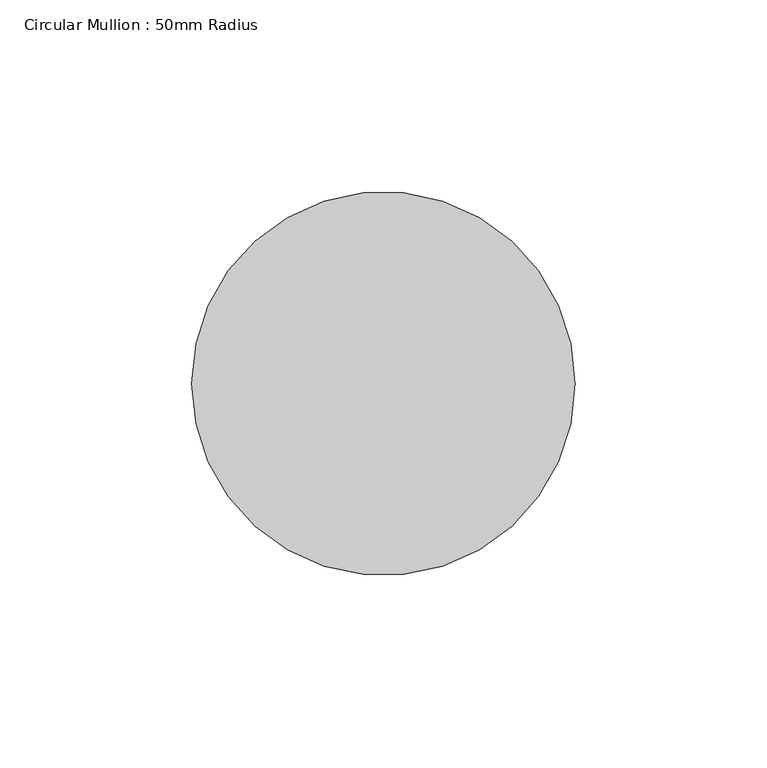
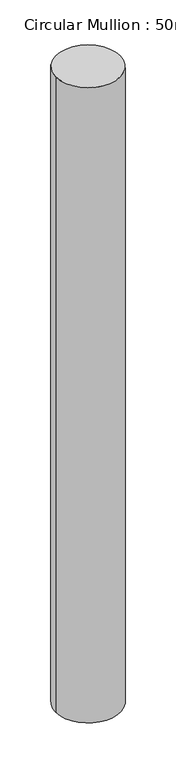
"""IFC4 building model written with IfcOpenShell, lengths in millimetres: member geometry, Circular Mullion : 50mm Radius."""

from ifc_helpers import new_model, si_unit, point, frame, origin, origin_2d, place, context, project, spatial, circle_curve, trimmed, segment, composite_curve, outline, extrude, source, transform, mapped, element, save


def circular_mullion_50mm_radius_1879a9a9(model_context):
    return source(origin(), model_context, "Body", "SweptSolid", [
        extrude(outline(composite_curve([segment(trimmed(circle_curve(origin_2d(), 50.0), [point((50.0, 0.0))], [point((-50.0, 0.0))], False, "CARTESIAN"), True, "CONTINUOUS"), segment(trimmed(circle_curve(origin_2d(), 50.0), [point((-50.0, 0.0))], [point((50.0, 0.0))], False, "CARTESIAN"), True, "CONTINUOUS")], self_intersect=False)), frame((0.0, 0.0, -1042.8045224), z_axis=(0.0, 0.0, 1.0), x_axis=(1.0, 0.0, 0.0)), (0.0, 0.0, 1.0), 1042.8045224),
    ])


if __name__ == "__main__":
    model = new_model("IFC4")
    model_context = context("Model", 3, world=origin())
    ifc_project = project(units=[si_unit("LENGTHUNIT", "METRE", prefix="MILLI")], contexts=[model_context])
    site = spatial("IfcSite", under=ifc_project)
    building = spatial("IfcBuilding", under=site)
    placement = place(None, origin())
    circular_mullion_50mm_radius_shape = circular_mullion_50mm_radius_1879a9a9(model_context)
    element("IfcMember", 1, ObjectType="Circular Mullion : 50mm Radius", at=placement, inside=building, context=model_context, shape_type="MappedRepresentation", body=[
        mapped(circular_mullion_50mm_radius_shape, transform((0.0, 0.0, 0.0), x_axis=(1.0, 0.0, 0.0), y_axis=(0.0, 1.0, 0.0), z_axis=(0.0, 0.0, 1.0))),
    ])
    save(model, "model.ifc")

# Revit data of these elements
# Type "Circular Mullion : 50mm Radius"
#   built-in parameter 1007350 = 0.164042 (stored number, unit not read)
# Element 1 (IfcMember, "Circular Mullion : 50mm Radius")
#   Materials on its faces: "Aluminium"
# Materials
#   "Aluminium": class "Metal", colour RGB 247 247 247, transparency 0, Description = "Aluminium 6061", Cost = 0
